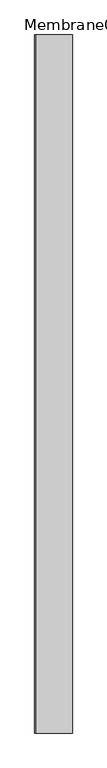
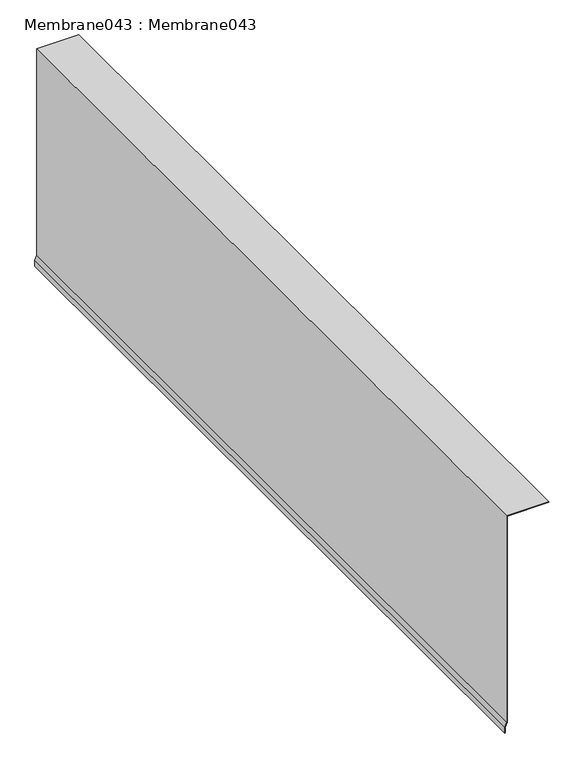
"""IFC4 building model written with IfcOpenShell, lengths in millimetres: proxy geometry, Membrane043 : Membrane043."""

from ifc_helpers import new_model, si_unit, frame, origin, place, context, project, spatial, polyline, outline, extrude, source, transform, mapped, element, save


def membrane043_membrane043_e69aa1f0(model_context):
    return source(origin(), model_context, "Body", "SweptSolid", [
        extrude(outline(polyline([(40115.330633, -9788.4545063), (40115.330633, -9892.1962891), (39579.4993977, -9892.1962891), (39568.2741325, -9896.2819515), (39552.6918208, -9896.2819515), (39552.6918208, -9895.2819515), (39568.0978055, -9895.2819515), (39579.3230707, -9891.1962891), (40114.330633, -9891.1962891), (40114.330633, -9788.4545063), (40115.330633, -9788.4545063)])), frame((0.0, 7182.1531721, 0.0), z_axis=(0.0, 1.0, 0.0), x_axis=(0.0, 0.0, 1.0)), (0.0, 0.0, 1.0), 2000.0),
    ])


if __name__ == "__main__":
    model = new_model("IFC4")
    model_context = context("Model", 3, world=origin())
    ifc_project = project(units=[si_unit("LENGTHUNIT", "METRE", prefix="MILLI")], contexts=[model_context])
    site = spatial("IfcSite", under=ifc_project)
    building = spatial("IfcBuilding", under=site)
    placement = place(None, origin())
    membrane043_membrane043_shape = membrane043_membrane043_e69aa1f0(model_context)
    element("IfcBuildingElementProxy", 1, Name="Membrane043 : Membrane043", ObjectType="Membrane043 : Membrane043", at=placement, inside=building, context=model_context, shape_type="MappedRepresentation", body=[
        mapped(membrane043_membrane043_shape, transform((0.0, 0.0, 0.0), x_axis=(1.0, 0.0, 0.0), y_axis=(0.0, 1.0, 0.0), z_axis=(0.0, 0.0, 1.0))),
    ])
    save(model, "model.ifc")

# Revit data of these elements
# Type "Membrane043 : Membrane043"
#   NameOverride = "Membrane043"
# Element 1 (IfcBuildingElementProxy, "Membrane043 : Membrane043")
#   Materials on its faces: "(2) LAYERS OF ICE & WATER SHIELD (BITUTHANE) UNDER STUCCO"
# Materials
#   "(2) LAYERS OF ICE & WATER SHIELD (BITUTHANE) UNDER STUCCO": class "Unassigned", colour RGB 186 255 159, transparency 0, Cost = 0
